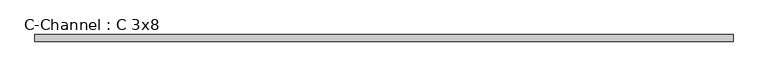
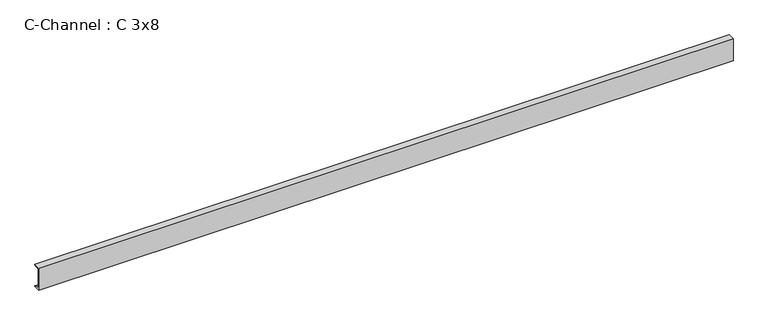
"""IFC4 building model written with IfcOpenShell, lengths in millimetres: beam geometry, C-Channel : C 3x8."""

from ifc_helpers import new_model, si_unit, point, frame, frame_2d, origin, place, context, project, spatial, polyline, circle_curve, trimmed, segment, composite_curve, outline, extrude, source, transform, mapped, element, save


def c_channel_c_3x8_0f191833(model_context):
    return source(origin(), model_context, "Body", "SweptSolid", [
        extrude(outline(composite_curve([segment(polyline([(-13.5128, 101.6), (44.9072, 101.6)]), True, "CONTINUOUS"), segment(trimmed(circle_curve(frame_2d((35.6108, 101.6)), 9.2964), [point((44.9072, 101.6))], [point((35.6108, 92.3036))], False, "CARTESIAN"), True, "CONTINUOUS"), segment(polyline([(35.6108, 92.3036), (-2.8702, 86.2088084), (-2.8702, -86.2088084), (35.6108, -92.3036)]), True, "CONTINUOUS"), segment(trimmed(circle_curve(frame_2d((35.6108, -101.6)), 9.2964), [point((35.6108, -92.3036))], [point((44.9072, -101.6))], False, "CARTESIAN"), True, "CONTINUOUS"), segment(polyline([(44.9072, -101.6), (-13.5128, -101.6), (-13.5128, 101.6)]), True, "CONTINUOUS")], self_intersect=False)), frame((-12252.325, 0.0, 0.0), z_axis=(1.0, 0.0, 0.0), x_axis=(0.0, 1.0, 0.0)), (0.0, 0.0, 1.0), 6108.7),
    ])


if __name__ == "__main__":
    model = new_model("IFC4")
    model_context = context("Model", 3, world=origin())
    ifc_project = project(units=[si_unit("LENGTHUNIT", "METRE", prefix="MILLI")], contexts=[model_context])
    site = spatial("IfcSite", under=ifc_project)
    building = spatial("IfcBuilding", under=site)
    placement = place(None, origin())
    c_channel_c_3x8_shape = c_channel_c_3x8_0f191833(model_context)
    element("IfcBeam", 1, ObjectType="C-Channel : C 3x8", at=placement, inside=building, context=model_context, shape_type="MappedRepresentation", body=[
        mapped(c_channel_c_3x8_shape, transform((0.0, 0.0, 0.0), x_axis=(1.0, 0.0, 0.0), y_axis=(0.0, 1.0, 0.0), z_axis=(0.0, 0.0, 1.0))),
    ])
    save(model, "model.ifc")

# Revit data of these elements
# Type "C-Channel : C 3x8"
#   Assembly Code = "B10"
#   W = 14.7
#   Length [instance default] = 5' - 0"
#   bf = 0' - 2.3"
#   d = 0' - 8"
#   tf = 0' - 0.366"
#   tw = 0' - 0.419"
#   x = 0' - 0.532"
#   A = 0.0300694 SF
#   Structural Material [instance default] = Steel ASTM A36
# Element 1 (IfcBeam, "C-Channel : C 3x8")
#   Structural Material = Steel ASTM A992
#   Materials on its faces: "Steel ASTM A992"
# Materials
#   "Steel ASTM A36": class "Metal", colour RGB 199 199 199, transparency 0, Description = "Structural steel, ASTM A36 Grade B, mill finish", Cost = 0
#   "Steel ASTM A992": class "Metal", colour RGB 189 187 185, transparency 0, Description = "Structural steel 50ksi", Cost = 0
